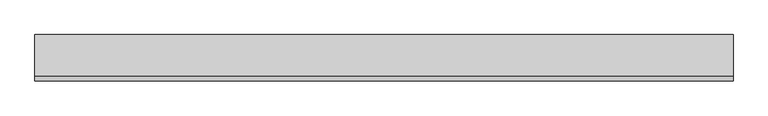
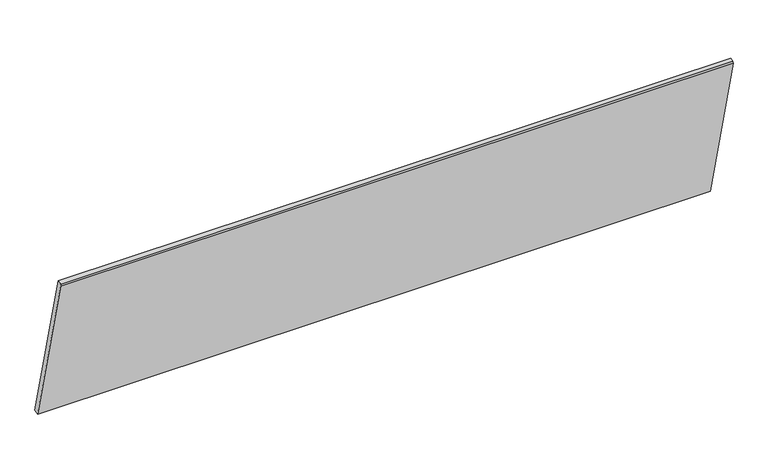
"""IFC4 building model written with IfcOpenShell, lengths in millimetres: proxy geometry, Gypsum008 919 : Gypsum008 919."""

from ifc_helpers import new_model, si_unit, frame, origin, place, context, project, spatial, polyline, outline, extrude, source, transform, mapped, element, save


def generic_models_d0d3208e(model_context):
    return source(origin(), model_context, "Body", "SweptSolid", [
        extrude(outline(polyline([(9752.047493, 43222.0071182), (9737.9368073, 43218.4770293), (9619.3816911, 43692.3727377), (9619.9854477, 43698.7661533), (9632.0226951, 43701.7775274), (9752.047493, 43222.0071182)])), frame((3694.2883192, 0.0, 0.0), z_axis=(1.0, 0.0, 0.0), x_axis=(0.0, 1.0, 0.0)), (0.0, 0.0, 1.0), 2000.0),
    ])


if __name__ == "__main__":
    model = new_model("IFC4")
    model_context = context("Model", 3, world=origin())
    ifc_project = project(units=[si_unit("LENGTHUNIT", "METRE", prefix="MILLI")], contexts=[model_context])
    site = spatial("IfcSite", under=ifc_project)
    building = spatial("IfcBuilding", under=site)
    placement = place(None, origin())
    generic_models_shape = generic_models_d0d3208e(model_context)
    element("IfcBuildingElementProxy", 1, Name="Gypsum008 919 : Gypsum008 919", ObjectType="Gypsum008 919 : Gypsum008 919", at=placement, inside=building, context=model_context, shape_type="MappedRepresentation", body=[
        mapped(generic_models_shape, transform((0.0, 0.0, 0.0), x_axis=(1.0, 0.0, 0.0), y_axis=(0.0, 1.0, 0.0), z_axis=(0.0, 0.0, 1.0))),
    ])
    save(model, "model.ifc")

# Revit data of these elements
# Type "Gypsum008 919 : Gypsum008 919"
#   NameOverride = "Gypsum008"
# Element 1 (IfcBuildingElementProxy, "Gypsum008 919 : Gypsum008 919")
#   Materials on its faces: "5/8\"  GYPSUM BOARD"
# Materials
#   "5/8\"  GYPSUM BOARD": class "Unassigned", colour RGB 255 255 255, transparency 0, Cost = 0
